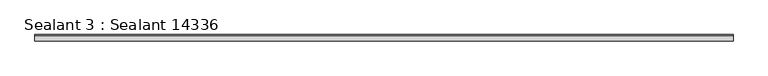
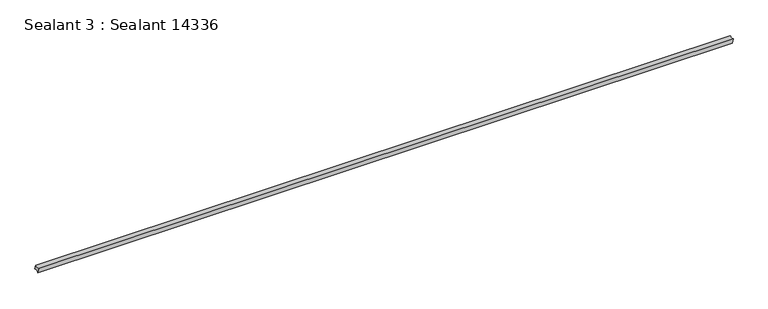
"""IFC4 building model written with IfcOpenShell, lengths in millimetres: proxy geometry, Sealant 3 : Sealant 14336."""

from ifc_helpers import new_model, si_unit, point, frame, frame_2d, origin, place, context, project, spatial, polyline, circle_curve, trimmed, segment, composite_curve, outline, extrude, source, transform, mapped, element, save


def sealant_3_sealant_14336_35b86830(model_context):
    return source(origin(), model_context, "Body", "SweptSolid", [
        extrude(outline(composite_curve([segment(polyline([(10812.8048921, 43495.8445422), (10816.7668382, 43483.0479011)]), True, "CONTINUOUS"), segment(trimmed(circle_curve(frame_2d((10811.0481461, 43475.0689569)), 9.816669), [point((10816.7668382, 43483.0479011))], [point((10802.0009766, 43478.8789063))], True, "CARTESIAN"), True, "CONTINUOUS"), segment(polyline([(10802.0009766, 43478.8789063), (10798.440969, 43495.2007936)]), True, "CONTINUOUS"), segment(trimmed(circle_curve(frame_2d((10805.3176151, 43502.3351513)), 9.9089516), [point((10798.440969, 43495.2007936))], [point((10812.8048921, 43495.8445422))], True, "CARTESIAN"), True, "CONTINUOUS")], self_intersect=False)), frame((3627.1902954, 0.0, 0.0), z_axis=(1.0, 0.0, 0.0), x_axis=(0.0, 1.0, 0.0)), (0.0, 0.0, 1.0), 1999.85),
    ])


if __name__ == "__main__":
    model = new_model("IFC4")
    model_context = context("Model", 3, world=origin())
    ifc_project = project(units=[si_unit("LENGTHUNIT", "METRE", prefix="MILLI")], contexts=[model_context])
    site = spatial("IfcSite", under=ifc_project)
    building = spatial("IfcBuilding", under=site)
    placement = place(None, origin())
    sealant_3_sealant_14336_shape = sealant_3_sealant_14336_35b86830(model_context)
    element("IfcBuildingElementProxy", 1, Name="Sealant 3 : Sealant 14336", ObjectType="Sealant 3 : Sealant 14336", at=placement, inside=building, context=model_context, shape_type="MappedRepresentation", body=[
        mapped(sealant_3_sealant_14336_shape, transform((0.0, 0.0, 0.0), x_axis=(1.0, 0.0, 0.0), y_axis=(0.0, 1.0, 0.0), z_axis=(0.0, 0.0, 1.0))),
    ])
    save(model, "model.ifc")

# Revit data of these elements
# Type "Sealant 3 : Sealant 14336"
#   NameOverride = "Sealant"
# Element 1 (IfcBuildingElementProxy, "Sealant 3 : Sealant 14336")
#   Materials on its faces: "SEALANT AND BACKER ROD WHERE NECESSARY"
# Materials
#   "SEALANT AND BACKER ROD WHERE NECESSARY": class "Unassigned", colour RGB 225 240 198, transparency 0, Cost = 0
